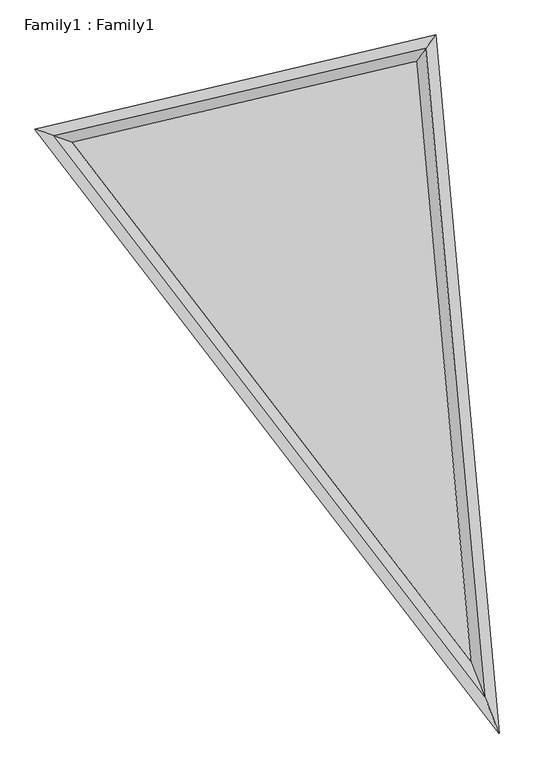
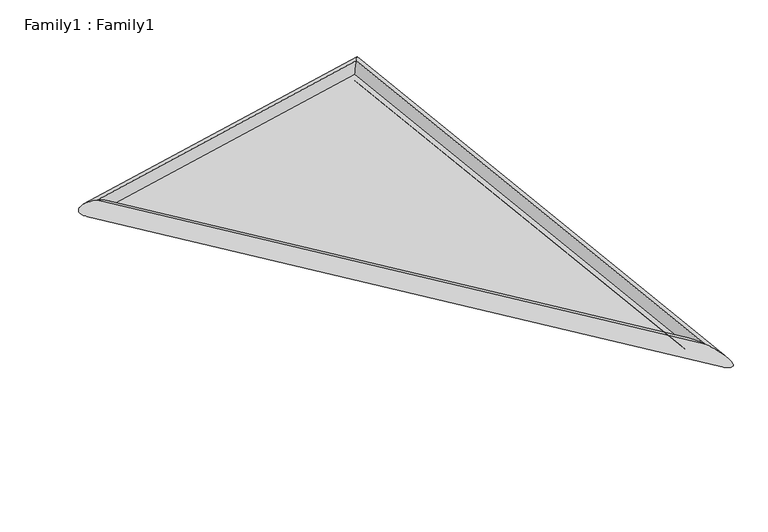
"""IFC4 building model written with IfcOpenShell, lengths in millimetres: proxy geometry, Family1 : Family1."""

from ifc_helpers import new_model, si_unit, frame, origin, origin_with_axes, place, context, project, spatial, polyline, ellipse_curve, outline, extrude, source, transform, mapped, element, save
from ifc_brep_helpers import cylinder_surface, advanced_brep


def family1_family1_a35ba392(model_context):
    return source(origin(), model_context, "Body", "SolidModel", [
        extrude(outline(polyline([(2414.5133011, -3219.5219796), (-1524.6901804, 1902.8178134), (1877.0993303, 2700.645371), (2414.5133011, -3219.5219796)])), origin_with_axes(), (0.0, 0.0, 1.0), 34.1328789),
        advanced_brep(
        [(2414.5133011, -3219.5219796, 100.0), (2414.5133011, -3219.5219796, -100.0), (-1524.6901804, 1902.8178134, -100.0), (-1524.6901804, 1902.8178134, 100.0), (1877.0993303, 2700.645371, -100.0), (1877.0993303, 2700.645371, 100.0)],
        [
            (0, 1, ellipse_curve(frame((2414.5133011, -3219.5219796, 0.0), z_axis=(-0.9312210746599368, -0.3644548121635832, 0.0), x_axis=(0.3644548121635831, -0.9312210746599366, 0.0)), 358.711881, 100.0)),
            (1, 2),
            (2, 3, ellipse_curve(frame((-1524.6901804, 1902.8178134, 0.0), z_axis=(-0.3357780914040767, -0.9419411198865009, 0.0), x_axis=(0.9419411198865009, -0.3357780914040769, 0.0)), 184.5063833, 100.0)),
            (3, 0),
            (1, 0, ellipse_curve(frame((2414.5133011, -3219.5219796, 0.0), z_axis=(-0.9312210746599368, -0.3644548121635832, 0.0), x_axis=(0.3644548121635831, -0.9312210746599366, 0.0)), 358.711881, 100.0)),
            (3, 2, ellipse_curve(frame((-1524.6901804, 1902.8178134, 0.0), z_axis=(-0.3357780914040767, -0.9419411198865009, 0.0), x_axis=(0.9419411198865009, -0.3357780914040769, 0.0)), 184.5063833, 100.0)),
            (2, 4),
            (4, 5, ellipse_curve(frame((1877.0993303, 2700.645371, 0.0), z_axis=(-0.8109925248626817, 0.5850565140367662, 0.0), x_axis=(-0.585056514036766, -0.8109925248626817, 0.0)), 152.4439953, 100.0)),
            (5, 3),
            (5, 4, ellipse_curve(frame((1877.0993303, 2700.645371, 0.0), z_axis=(-0.8109925248626817, 0.5850565140367662, 0.0), x_axis=(-0.585056514036766, -0.8109925248626817, 0.0)), 152.4439953, 100.0)),
            (4, 1),
            (0, 5),
        ],
        [
            cylinder_surface(frame((2414.5133011, -3219.5219796, 0.0), z_axis=(0.6096079019368956, -0.79270310072315, 0.0), x_axis=(-0.79270310072315, -0.6096079019368956, 0.0)), 100.0),
            cylinder_surface(frame((-1524.6901804, 1902.8178134, 0.0), z_axis=(-0.9735824002451955, -0.22833595847523405, 0.0), x_axis=(-0.22833595847523405, 0.9735824002451955, 0.0)), 100.0),
            cylinder_surface(frame((1877.0993303, 2700.645371, 0.0), z_axis=(-0.09040509656049721, 0.9959050750527819, 0.0), x_axis=(0.9959050750527819, 0.09040509656049721, 0.0)), 100.0),
        ],
        [
            (0, [[1, 2, 3, 4]]),
            (0, [[5, -4, 6, -2]]),
            (1, [[-3, 7, 8, 9]]),
            (1, [[-6, -9, 10, -7]]),
            (2, [[-8, 11, -1, 12]]),
            (2, [[-10, -12, -5, -11]]),
        ],
    ),
    ])


if __name__ == "__main__":
    model = new_model("IFC4")
    model_context = context("Model", 3, world=origin())
    ifc_project = project(units=[si_unit("LENGTHUNIT", "METRE", prefix="MILLI")], contexts=[model_context])
    site = spatial("IfcSite", under=ifc_project)
    building = spatial("IfcBuilding", under=site)
    placement = place(None, origin())
    family1_family1_shape = family1_family1_a35ba392(model_context)
    element("IfcBuildingElementProxy", 1, Name="Family1 : Family1", ObjectType="Family1 : Family1", at=placement, inside=building, context=model_context, shape_type="MappedRepresentation", body=[
        mapped(family1_family1_shape, transform((0.0, 0.0, 0.0), x_axis=(1.0, 0.0, 0.0), y_axis=(0.0, 1.0, 0.0), z_axis=(0.0, 0.0, 1.0))),
    ])
    save(model, "model.ifc")

# Revit data of these elements
# Type "Family1 : Family1"
#   Default Elevation = 0
# Element 1 (IfcBuildingElementProxy, "Family1 : Family1")
#   Materials on its faces: "Glass"
# Materials
#   "Glass": class "Glass", colour RGB 0 128 192, transparency 0.9, Description = "Soda Lime Glass", Cost = 0
